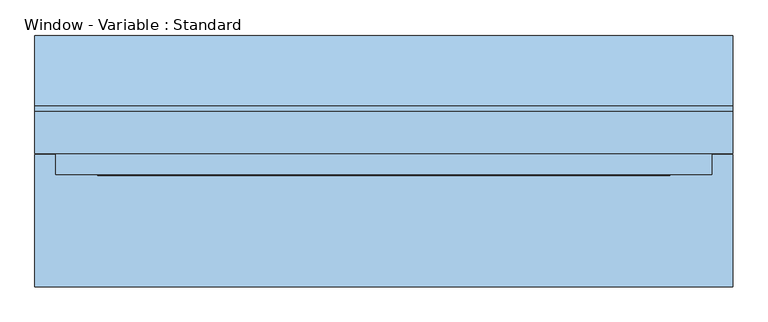
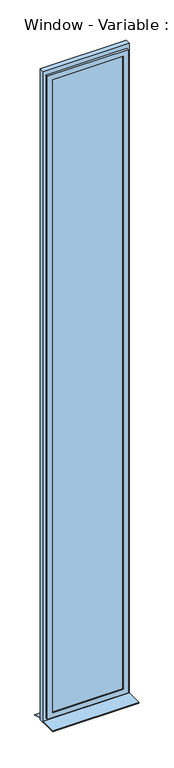
"""IFC4 building model written with IfcOpenShell, lengths in millimetres: window geometry, Window - Variable : Standard."""

from ifc_helpers import new_model, si_unit, frame, origin, place, context, project, spatial, polyline, outline, extrude, faceted_brep, source, transform, mapped, element, save


def window_variable_standard_7c8c74e5(model_context):
    return source(origin(), model_context, "Body", "SolidModel", [
        extrude(outline(polyline([(9000.0, 500.0), (9000.0, -500.0), (1000.0, -500.0), (1000.0, 500.0), (9000.0, 500.0)]), holes=[polyline([(8920.0, 440.0), (1080.0, 440.0), (1080.0, -440.0), (8920.0, -440.0), (8920.0, 440.0)])]), frame((0.0, 10.0, 0.0), z_axis=(0.0, 1.0, 0.0), x_axis=(0.0, 0.0, 1.0)), (0.0, 0.0, 1.0), 60.0),
        faceted_brep([(470.0, 10.0, 8950.0), (470.0, -20.0, 8950.0), (470.0, -20.0, 1050.0), (470.0, 10.0, 1050.0), (-470.0, -20.0, 8950.0), (-470.0, -20.0, 1050.0), (410.0, -20.0, 1110.0), (-410.0, -20.0, 1110.0), (-410.0, -20.0, 8890.0), (410.0, -20.0, 8890.0), (-470.0, 10.0, 1050.0), (-470.0, 10.0, 8950.0), (440.0, 10.0, 8920.0), (-440.0, 10.0, 8920.0), (-440.0, 10.0, 1080.0), (440.0, 10.0, 1080.0), (440.0, 40.0, 8920.0), (440.0, 40.0, 1080.0), (-440.0, 40.0, 1080.0), (-440.0, 40.0, 8920.0), (410.0, 40.0, 8890.0), (-410.0, 40.0, 8890.0), (-410.0, 40.0, 1110.0), (410.0, 40.0, 1110.0)], [[[0, 1, 2, 3]], [[1, 4, 5, 2], [6, 7, 8, 9]], [[3, 2, 5, 10]], [[3, 10, 11, 0], [12, 13, 14, 15]], [[16, 12, 15, 17]], [[17, 15, 14, 18]], [[17, 18, 19, 16], [20, 21, 22, 23]], [[9, 20, 23, 6]], [[6, 23, 22, 7]], [[10, 5, 4, 11]], [[18, 14, 13, 19]], [[7, 22, 21, 8]], [[11, 4, 1, 0]], [[19, 13, 12, 16]], [[8, 21, 20, 9]]]),
        extrude(outline(polyline([(-500.0, -180.0), (-500.0, 10.0), (500.0, 10.0), (500.0, -180.0), (-500.0, -180.0)])), frame((0.0, 0.0, 1005.0), z_axis=(0.0, 0.0, 1.0), x_axis=(1.0, 0.0, 0.0)), (0.0, 0.0, 1.0), 15.0),
        extrude(outline(polyline([(80.0221543, 1020.0), (180.0, 1000.0), (180.0, 990.0), (178.0, 990.0), (178.0, 998.3604634), (79.8240723, 1018.0), (70.0, 1018.0), (70.0, 1020.0), (80.0221543, 1020.0)])), frame((-500.0, 0.0, 0.0), z_axis=(1.0, 0.0, 0.0), x_axis=(0.0, 1.0, 0.0)), (0.0, 0.0, 1.0), 1000.0),
        extrude(outline(polyline([(410.0, -5.0), (-410.0, -5.0), (-410.0, 25.0), (410.0, 25.0), (410.0, -5.0)])), frame((0.0, 0.0, 1110.0), z_axis=(0.0, 0.0, 1.0), x_axis=(1.0, 0.0, 0.0)), (0.0, 0.0, 1.0), 7780.0),
    ])


if __name__ == "__main__":
    model = new_model("IFC4")
    model_context = context("Model", 3, world=origin())
    ifc_project = project(units=[si_unit("LENGTHUNIT", "METRE", prefix="MILLI")], contexts=[model_context])
    site = spatial("IfcSite", under=ifc_project)
    building = spatial("IfcBuilding", under=site)
    placement = place(None, origin())
    window_variable_standard_shape = window_variable_standard_7c8c74e5(model_context)
    element("IfcWindow", 1, ObjectType="Window - Variable : Standard", at=placement, inside=building, context=model_context, shape_type="MappedRepresentation", body=[
        mapped(window_variable_standard_shape, transform((0.0, 0.0, 0.0), x_axis=(1.0, 0.0, 0.0), y_axis=(0.0, 1.0, 0.0), z_axis=(0.0, 0.0, 1.0))),
    ])
    save(model, "model.ifc")

# Revit data of these elements
# Type "Window - Variable : Standard"
#   Type Mark = "19"
#   Operation = "SinglePanel"
#   Keynote = "16.05.01"
#   Analytic Construction = "<None>"
#   Rough Width [instance default] = 1.010 m
#   Rough Height [instance default] = 1.010 m
#   Frame Depth = 0.060 m
#   Frame Height Bottom = 0.080 m
#   Frame Height Top = 0.080 m
#   Frame Width = 0.060 m
#   Height [instance default] = 1.010 m
#   Window Inset = 0.060 m
#   Window Width = 0.060 m
#   Instalation Depth [instance default] = 0.080 m
#   Width [instance default] = 1.010 m
#   Folding Wing [instance default] = no
#   Oppening Direction Vertical [instance default] = yes
#   Oppening Direction Visibility [instance default] = no
#   Casement [instance default] = yes
#   Frame [instance default] = none
#   Glas [instance default] = none
#   Window [instance default] = none
#   Windowsill Inside [instance default] = none
#   Windowsill Outside [instance default] = none
#   Wall Closure = (empty or 0)
#   Assembly Code = ""
# Element 1 (IfcWindow, "Window - Variable : Standard")
#   Rough Width = 1.000 m
#   Rough Height = 8.000 m
#   Height = 8.000 m
#   Width = 1.000 m
#   Materials on its faces: "Plastic - White", "Metal _ Aluminium", "Wood - Birch", "Glass"
# Materials
#   "Plastic - White": class "Kunststoff", colour RGB 249 249 249, transparency 0
#   "Metal _ Aluminium": class "Metall", colour RGB 247 247 247, transparency 0
#   "Wood - Birch": class "Holz", colour RGB 213 164 103, transparency 0
#   "Glass": class "Glass", colour RGB 0 128 192, transparency 0.9
